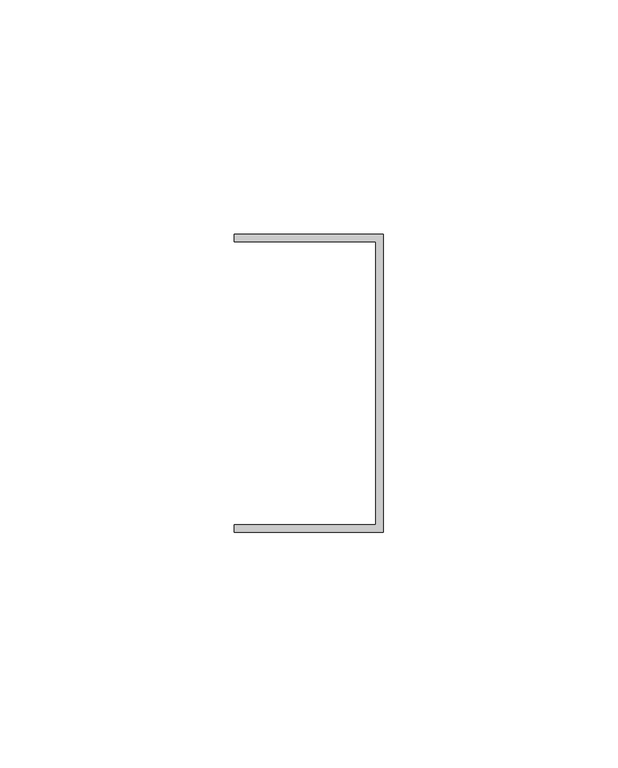
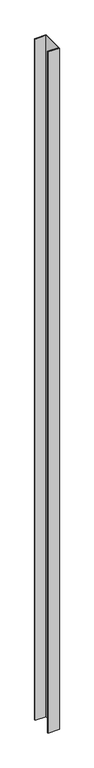
"""IFC4 building model written with IfcOpenShell, lengths in millimetres: proxy geometry, Generic Models 7:Generic Models 1:3:Generic Models 1:3 : Generic Models 7:Generic Models 1:305549:3:Generic Models 1:3:Generic Models 1:3 : Generic Models 7:Generic Models 1:305549:3 : Generic Models 7:Generic Models 1:3:Generic Models 1:3 : Generic Models 7:Generic Models 1:305549:301244:8 : Generic Models 7:Generic Models 1:3:Generic Models 1:3 : Generic Models 7:Generic Models 1:305549:3:Generic Models 1:3:Generic Models 1:3 : Generic Models 7:Generic Models 1:305549:3 : Generic Models 7:Generic Models 1:3:Generic Models 1:3 : Generic Models 7:Generic Models 1:305549:301244:308848."""

from ifc_helpers import new_model, si_unit, frame, origin, place, context, project, spatial, polyline, outline, extrude, source, transform, mapped, element, save


def generic_models_3a56f2cc(model_context):
    return source(origin(), model_context, "Body", "SweptSolid", [
        extrude(outline(polyline([(560635.536724, -579013.3913841), (560635.536724, -579076.8913841), (560603.786724, -579076.8913841), (560603.786724, -579075.3038841), (560633.949224, -579075.3038841), (560633.949224, -579014.9788841), (560603.786724, -579014.9788841), (560603.786724, -579013.3913841), (560635.536724, -579013.3913841)])), frame((0.0, 0.0, 4133.81326), z_axis=(0.0, 0.0, 1.0), x_axis=(1.0, 0.0, 0.0)), (0.0, 0.0, 1.0), 2000.28674),
    ])


if __name__ == "__main__":
    model = new_model("IFC4")
    model_context = context("Model", 3, world=origin())
    ifc_project = project(units=[si_unit("LENGTHUNIT", "METRE", prefix="MILLI")], contexts=[model_context])
    site = spatial("IfcSite", under=ifc_project)
    building = spatial("IfcBuilding", under=site)
    placement = place(None, origin())
    generic_models_shape = generic_models_3a56f2cc(model_context)
    element("IfcBuildingElementProxy", 1, Name="Generic Models 7:Generic Models 1:3:Generic Models 1:3 : Generic Models 7:Generic Models 1:305549:3:Generic Models 1:3:Generic Models 1:3 : Generic Models 7:Generic Models 1:305549:3 : Generic Models 7:Generic Models 1:3:Generic Models 1:3 : Generic Models 7:Generic Models 1:305549:301244:8 : Generic Models 7:Generic Models 1:3:Generic Models 1:3 : Generic Models 7:Generic Models 1:305549:3:Generic Models 1:3:Generic Models 1:3 : Generic Models 7:Generic Models 1:305549:3 : Generic Models 7:Generic Models 1:3:Generic Models 1:3 : Generic Models 7:Generic Models 1:305549:301244:308848", ObjectType="Generic Models 7:Generic Models 1:3:Generic Models 1:3 : Generic Models 7:Generic Models 1:305549:3:Generic Models 1:3:Generic Models 1:3 : Generic Models 7:Generic Models 1:305549:3 : Generic Models 7:Generic Models 1:3:Generic Models 1:3 : Generic Models 7:Generic Models 1:305549:301244:8 : Generic Models 7:Generic Models 1:3:Generic Models 1:3 : Generic Models 7:Generic Models 1:305549:3:Generic Models 1:3:Generic Models 1:3 : Generic Models 7:Generic Models 1:305549:3 : Generic Models 7:Generic Models 1:3:Generic Models 1:3 : Generic Models 7:Generic Models 1:305549:301244:308848", at=placement, inside=building, context=model_context, shape_type="MappedRepresentation", body=[
        mapped(generic_models_shape, transform((0.0, 0.0, 0.0), x_axis=(1.0, 0.0, 0.0), y_axis=(0.0, 1.0, 0.0), z_axis=(0.0, 0.0, 1.0))),
    ])
    save(model, "model.ifc")

# Revit data of these elements
# Type "Generic Models 7:Generic Models 1:3:Generic Models 1:3 : Generic Models 7:Generic Models 1:305549:3:Generic Models 1:3:Generic Models 1:3 : Generic Models 7:Generic Models 1:305549:3 : Generic Models 7:Generic Models 1:3:Generic Models 1:3 : Generic Models 7:Generic Models 1:305549:301244:8 : Generic Models 7:Generic Models 1:3:Generic Models 1:3 : Generic Models 7:Generic Models 1:305549:3:Generic Models 1:3:Generic Models 1:3 : Generic Models 7:Generic Models 1:305549:3 : Generic Models 7:Generic Models 1:3:Generic Models 1:3 : Generic Models 7:Generic Models 1:305549:301244:308848"
#   NameOverride = "Generic Models 7:Generic Models 1:3:Generic Models 1:3 : Generic Models 7:Generic Models 1:305549:3:Generic Models 1:3:Generic Models 1:3 : Generic Models 7:Generic Models 1:305549:3 : Generic Models 7:Generic Models 1:3:Generic Models 1:3 : Generic Models 7:Generic Models 1:305549:301244:308848"
#   ObjectTypeOverride = "Generic Models 1:3:Generic Models 1:3 : Generic Models 7:Generic Models 1:305549:3 : Generic Models 7:Generic Models 1:3:Generic Models 1:3 : Generic Models 7:Generic Models 1:305549:301244"
#   Reference = "Generic Models 1"
#   Tag = "308848"
# Element 1 (IfcBuildingElementProxy, "Generic Models 7:Generic Models 1:3:Generic Models 1:3 : Generic Models 7:Generic Models 1:305549:3:Generic Models 1:3:Generic Models 1:3 : Generic Models 7:Generic Models 1:305549:3 : Generic Models 7:Generic Models 1:3:Generic Models 1:3 : Generic Models 7:Generic Models 1:305549:301244:8 : Generic Models 7:Generic Models 1:3:Generic Models 1:3 : Generic Models 7:Generic Models 1:305549:3:Generic Models 1:3:Generic Models 1:3 : Generic Models 7:Generic Models 1:305549:3 : Generic Models 7:Generic Models 1:3:Generic Models 1:3 : Generic Models 7:Generic Models 1:305549:301244:308848")
#   Materials on its faces: "GALVANIZED U-CHANNEL (250T125-33)"
# Materials
#   "GALVANIZED U-CHANNEL (250T125-33)": class "Unassigned", colour RGB 202 201 200, transparency 0, Keynote = "M05451300.02", Cost = 0
